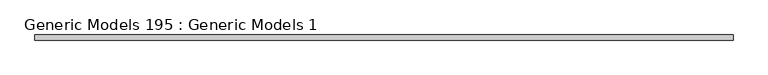
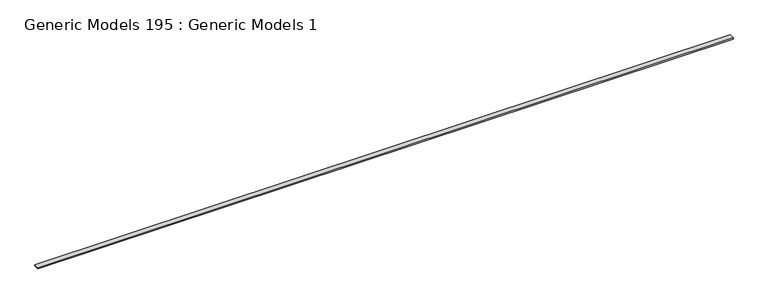
"""IFC4 building model written with IfcOpenShell, lengths in millimetres: proxy geometry, Generic Models 195 : Generic Models 1."""

from ifc_helpers import new_model, si_unit, frame, origin, place, context, project, spatial, polyline, outline, extrude, source, transform, mapped, element, save


def generic_models_195_generic_models_1_d685f574(model_context):
    return source(origin(), model_context, "Body", "SweptSolid", [
        extrude(outline(polyline([(-20998.9733045, -25331.0674751), (-20998.9733045, -25191.3674751), (-1948.9733045, -25191.3674751), (-1948.9733045, -25331.0674751), (-20998.9733045, -25331.0674751)])), frame((0.0, 0.0, 127066.3735933), z_axis=(0.0, 0.0, 1.0), x_axis=(1.0, 0.0, 0.0)), (0.0, 0.0, 1.0), 38.1),
    ])


if __name__ == "__main__":
    model = new_model("IFC4")
    model_context = context("Model", 3, world=origin())
    ifc_project = project(units=[si_unit("LENGTHUNIT", "METRE", prefix="MILLI")], contexts=[model_context])
    site = spatial("IfcSite", under=ifc_project)
    building = spatial("IfcBuilding", under=site)
    placement = place(None, origin())
    generic_models_195_generic_models_1_shape = generic_models_195_generic_models_1_d685f574(model_context)
    element("IfcBuildingElementProxy", 1, Name="Generic Models 195 : Generic Models 1", ObjectType="Generic Models 195 : Generic Models 1", at=placement, inside=building, context=model_context, shape_type="MappedRepresentation", body=[
        mapped(generic_models_195_generic_models_1_shape, transform((0.0, 0.0, 0.0), x_axis=(1.0, 0.0, 0.0), y_axis=(0.0, 1.0, 0.0), z_axis=(0.0, 0.0, 1.0))),
    ])
    save(model, "model.ifc")

# Revit data of these elements
# Element 1 (IfcBuildingElementProxy, "Generic Models 195 : Generic Models 1")
#   Materials on its faces: "_2X BLOCKING AS REQUIRED"
# Materials
#   "_2X BLOCKING AS REQUIRED": class "Generic", colour RGB 177 130 114, transparency 0, Cost = 0
